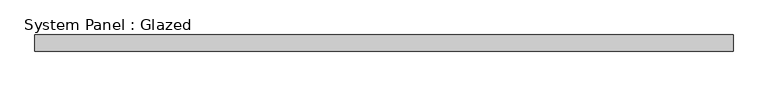
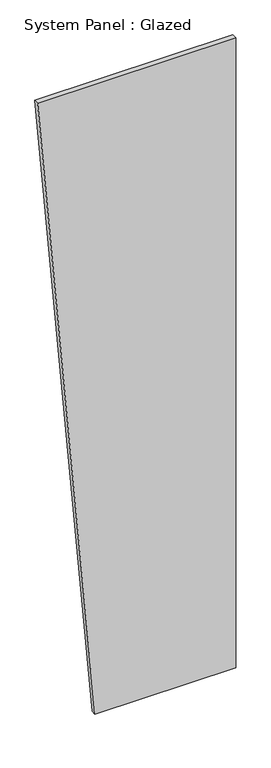
"""IFC4 building model written with IfcOpenShell, lengths in millimetres: plate geometry, System Panel : Glazed."""

import ifcopenshell
import ifcopenshell.guid

model = None  # the IFC model being written
_history = None  # IfcOwnerHistory: only IFC2X3 demands one
_inside = {}  # id of a spatial element -> (the spatial element, [elements in it])
_under = {}  # id of a project, library or spatial element -> (it, [spatial elements below it])
_declared = {}  # id of a project -> (the project, [libraries it declares])
_typed = {}  # id of a type object -> (the type object, [elements of that type])
_made_of = {}  # id of a material, layer set ... -> (it, [elements and type objects made of it])


def new_model(schema):
    """Start an empty IFC model of exactly this schema.

    Asked for "IFC4X3", IfcOpenShell would pick the latest addendum, in which some entities
    have other attributes; the version numbers below select the first issue.
    IFC2X3 requires an IfcOwnerHistory on every rooted entity: one is made here for all.
    """
    global model, _history
    if schema == "IFC4X3":
        model = ifcopenshell.file(schema_version=(4, 3, 0, 0))
    else:
        model = ifcopenshell.file(schema=schema)
    _inside.clear()
    _under.clear()
    _declared.clear()
    _typed.clear()
    _made_of.clear()
    _history = None
    if model.schema == "IFC2X3":
        org = make("IfcOrganization", Name="unknown")
        user = make(
            "IfcPersonAndOrganization",
            ThePerson=make("IfcPerson", FamilyName="unknown"),
            TheOrganization=org,
        )
        app = make(
            "IfcApplication",
            ApplicationDeveloper=org,
            Version="unknown",
            ApplicationFullName="unknown",
            ApplicationIdentifier="unknown",
        )
        _history = make(
            "IfcOwnerHistory",
            OwningUser=user,
            OwningApplication=app,
            ChangeAction="ADDED",
            CreationDate=0,
        )
    return model


def make(cls, **values):
    """One entity of the class cls with the attributes given. An attribute that is None is left unset."""
    return model.create_entity(
        cls, **{name: value for name, value in values.items() if value is not None}
    )


def rooted(cls, **values):
    """An entity with a GlobalId (a new one), such as an element, a storey or a relation."""
    return make(cls, GlobalId=ifcopenshell.guid.new(), OwnerHistory=_history, **values)


def si_unit(unit_type, name, prefix=None):
    """IfcSIUnit, for example si_unit("LENGTHUNIT", "METRE", prefix="MILLI")."""
    return make("IfcSIUnit", UnitType=unit_type, Prefix=prefix, Name=name)


def assignment(units):
    """IfcUnitAssignment: the units of a project."""
    return None if units is None else make("IfcUnitAssignment", Units=units)


def point(xyz):
    """IfcCartesianPoint."""
    return None if xyz is None else make("IfcCartesianPoint", Coordinates=xyz)


def direction(xyz):
    """IfcDirection."""
    return None if xyz is None else make("IfcDirection", DirectionRatios=xyz)


def frame(location, z_axis=None, x_axis=None):
    """IfcAxis2Placement3D, a coordinate frame: its origin and axes. An axis left out is left unset."""
    return make(
        "IfcAxis2Placement3D",
        Location=point(location),
        Axis=direction(z_axis),
        RefDirection=direction(x_axis),
    )


def origin():
    """The frame at (0, 0, 0) with its axes left unset."""
    return frame((0.0, 0.0, 0.0))


def place(relative_to, where):
    """IfcLocalPlacement: puts the frame where relative to a parent placement (None: the world)."""
    return make(
        "IfcLocalPlacement", PlacementRelTo=relative_to, RelativePlacement=where
    )


def context(
    kind, dimensions, precision=None, world=None, true_north=None, identifier=None
):
    """IfcGeometricRepresentationContext, for example the 3D "Model" context."""
    return make(
        "IfcGeometricRepresentationContext",
        ContextIdentifier=identifier,
        ContextType=kind,
        CoordinateSpaceDimension=dimensions,
        Precision=precision,
        WorldCoordinateSystem=world,
        TrueNorth=true_north,
    )


def project(units=None, contexts=None):
    """IfcProject with its units and contexts."""
    return rooted(
        "IfcProject",
        Name="project",
        RepresentationContexts=contexts,
        UnitsInContext=assignment(units),
    )


def spatial(cls, under=None, at=None, **own):
    """A site, building, storey or space (cls), placed at a placement, below another one or the project."""
    s = rooted(cls, ObjectPlacement=at, **own)
    if under is not None:
        _under.setdefault(under.id(), (under, []))[1].append(s)
    return s


def polyline(points):
    """IfcPolyline through the points."""
    return make("IfcPolyline", Points=[point(p) for p in points])


def outline(outer, holes=None, kind="AREA"):
    """IfcArbitraryClosedProfileDef: a profile drawn as a closed curve; with holes, ...WithVoids."""
    if holes is None:
        return make("IfcArbitraryClosedProfileDef", ProfileType=kind, OuterCurve=outer)
    return make(
        "IfcArbitraryProfileDefWithVoids",
        ProfileType=kind,
        OuterCurve=outer,
        InnerCurves=holes,
    )


def extrude(swept, where, along, depth):
    """IfcExtrudedAreaSolid: the profile swept, set in the frame where, extruded along a direction by depth."""
    return make(
        "IfcExtrudedAreaSolid",
        SweptArea=swept,
        Position=where,
        ExtrudedDirection=direction(along),
        Depth=depth,
    )


def shape(context_of_items, identifier, shape_type, items):
    """IfcShapeRepresentation: the items that make up one representation, for example the "Body"."""
    return make(
        "IfcShapeRepresentation",
        ContextOfItems=context_of_items,
        RepresentationIdentifier=identifier,
        RepresentationType=shape_type,
        Items=items,
    )


def source(mapping_origin, context_of_items, identifier, shape_type, items):
    """IfcRepresentationMap: a shape defined once, which mapped items show again and again."""
    return make(
        "IfcRepresentationMap",
        MappingOrigin=mapping_origin,
        MappedRepresentation=shape(context_of_items, identifier, shape_type, items),
    )


def transform(
    local_origin,
    x_axis=None,
    y_axis=None,
    z_axis=None,
    scale=None,
    scale2=None,
    scale3=None,
    uniform=True,
):
    """IfcCartesianTransformationOperator3D, or its non-uniform kind. x_axis, y_axis, z_axis: its Axis1, 2, 3."""
    if uniform:
        return make(
            "IfcCartesianTransformationOperator3D",
            Axis1=direction(x_axis),
            Axis2=direction(y_axis),
            LocalOrigin=point(local_origin),
            Scale=scale,
            Axis3=direction(z_axis),
        )
    return make(
        "IfcCartesianTransformationOperator3DnonUniform",
        Axis1=direction(x_axis),
        Axis2=direction(y_axis),
        LocalOrigin=point(local_origin),
        Scale=scale,
        Axis3=direction(z_axis),
        Scale2=scale2,
        Scale3=scale3,
    )


def mapped(mapping_source, mapping_target):
    """IfcMappedItem: shows the shape of a source again, moved by a transform."""
    return make(
        "IfcMappedItem", MappingSource=mapping_source, MappingTarget=mapping_target
    )


def made_of(thing, what):
    """Note that an element or type object is made of a material, layer set ...; save() writes the relation."""
    if what is not None:
        _made_of.setdefault(what.id(), (what, []))[1].append(thing)
    return thing


def element(
    cls,
    number,
    at=None,
    inside=None,
    cuts=None,
    type_object=None,
    material=None,
    context=None,
    identifier="Body",
    shape_type=None,
    held_by="IfcProductDefinitionShape",
    body=None,
    shapes=None,
    **own,
):
    """One element of the class cls, such as IfcWall. Its Tag is "e" and its number.

    at: its placement. inside: the storey or other place that contains it. cuts: it is an
    opening in that element (IfcRelVoidsElement). A single representation is given by context,
    identifier, shape_type and body (its items); several are given by shapes. held_by: the class
    of the entity that holds the representations. save() writes the other relations.
    """
    e = rooted(cls, Tag="e%d" % number, ObjectPlacement=at, **own)
    if body is not None:
        shapes = [shape(context, identifier, shape_type, body)]
    if shapes is not None:
        e.Representation = make(held_by, Representations=shapes)
    if inside is not None:
        _inside.setdefault(inside.id(), (inside, []))[1].append(e)
    if cuts is not None:
        rooted(
            "IfcRelVoidsElement", RelatingBuildingElement=cuts, RelatedOpeningElement=e
        )
    if type_object is not None:
        _typed.setdefault(type_object.id(), (type_object, []))[1].append(e)
    return made_of(e, material)


def aggregate(whole, parts):
    """IfcRelAggregates: a whole, such as a stair, and the parts it consists of."""
    return rooted("IfcRelAggregates", RelatingObject=whole, RelatedObjects=parts)


def save(model, path):
    """Write the relations noted so far, then the file.

    IfcRelAggregates (storeys below a building ...), IfcRelContainedInSpatialStructure (elements
    in a storey), IfcRelDefinesByType, IfcRelAssociatesMaterial and IfcRelDeclares: one each for
    every whole, place, type object, material and project.
    """
    for whole, parts in _under.values():
        aggregate(whole, parts)
    for where, things in _inside.values():
        rooted(
            "IfcRelContainedInSpatialStructure",
            RelatedElements=things,
            RelatingStructure=where,
        )
    for kind, things in _typed.values():
        rooted("IfcRelDefinesByType", RelatedObjects=things, RelatingType=kind)
    for what, things in _made_of.values():
        rooted("IfcRelAssociatesMaterial", RelatedObjects=things, RelatingMaterial=what)
    for by, libraries in _declared.values():
        rooted("IfcRelDeclares", RelatingContext=by, RelatedDefinitions=libraries)
    model.write(path)


def system_panel_glazed_d5b9b34d(model_context):
    return source(origin(), model_context, "Body", "SweptSolid", [
        extrude(outline(polyline([(0.0, -228.6), (0.0, 543.7370389), (3657.6, 543.7370389), (3657.6, -543.7370389), (0.0, -228.6)])), frame((0.0, -44.45, 0.0), z_axis=(0.0, 1.0, 0.0), x_axis=(0.0, 0.0, 1.0)), (0.0, 0.0, 1.0), 25.4),
    ])


if __name__ == "__main__":
    model = new_model("IFC4")
    model_context = context("Model", 3, world=origin())
    ifc_project = project(units=[si_unit("LENGTHUNIT", "METRE", prefix="MILLI")], contexts=[model_context])
    site = spatial("IfcSite", under=ifc_project)
    building = spatial("IfcBuilding", under=site)
    placement = place(None, origin())
    system_panel_glazed_shape = system_panel_glazed_d5b9b34d(model_context)
    element("IfcPlate", 1, ObjectType="System Panel : Glazed", at=placement, inside=building, context=model_context, shape_type="MappedRepresentation", body=[
        mapped(system_panel_glazed_shape, transform((0.0, 0.0, 0.0), x_axis=(1.0, 0.0, 0.0), y_axis=(0.0, 1.0, 0.0), z_axis=(0.0, 0.0, 1.0))),
    ])
    save(model, "model.ifc")

# Revit data of these elements
# Type "System Panel : Glazed"
#   Construction Type Id = "GSP4R"
#   Analytic Construction = "1/8 in Pilkington single glazing"
#   Visual Light Transmittance = 0.9
#   Solar Heat Gain Coefficient = 0.86
#   Heat Transfer Coefficient (U) = 1.18115 BTU/(h·ft²·°F)
#   Define Thermal Properties by = 1
# Element 1 (IfcPlate, "System Panel : Glazed")
#   Materials on its faces: "Glass"
# Materials
#   "Glass": class "Glass", colour RGB 0 128 192, transparency 0.75, Description = "Soda Lime Glass", Cost = 0
